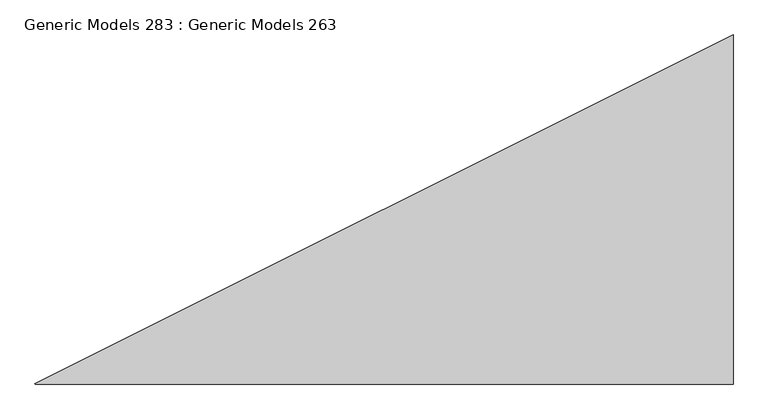
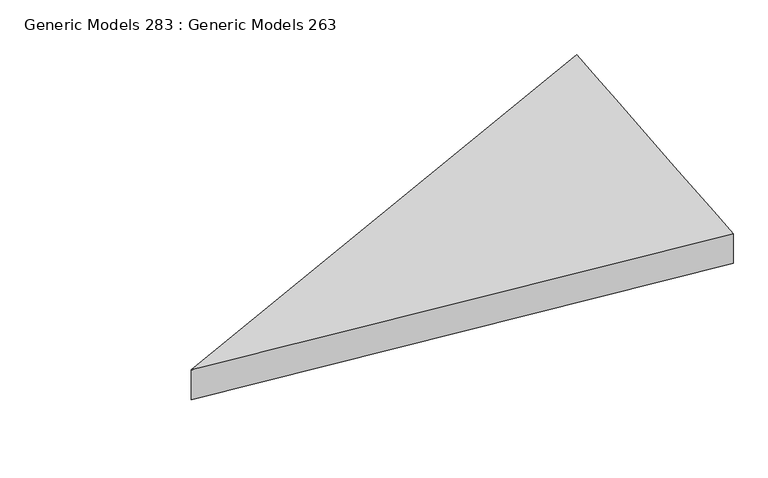
"""IFC4 building model written with IfcOpenShell, lengths in millimetres: proxy geometry, Generic Models 283 : Generic Models 263."""

from ifc_helpers import new_model, si_unit, frame, origin, place, context, project, spatial, source, transform, mapped, element, save
from ifc_brep_helpers import plane_surface, spline_surface, advanced_brep


def generic_models_283_generic_models_263_0de525de(model_context):
    return source(origin(), model_context, "Body", "AdvancedBrep", [
        advanced_brep(
        [(91554.5797726, 2106.5727422, 2.0699085), (91554.5797726, 582.5727422, -137.0198762), (91554.5797726, 582.5727422, -314.8198762), (91554.5797726, 2106.5727422, -314.8198762), (88506.5797726, 583.7192284, 120.3150753), (88506.5797726, 583.7192284, -58.1173502), (88506.5797726, 582.5727422, -58.1173502), (88506.5797726, 582.5727422, 120.3150753)],
        [
            (0, 1),
            (1, 2),
            (2, 3),
            (3, 0),
            (4, 5),
            (5, 6),
            (6, 7),
            (7, 4),
            (4, 0),
            (3, 5),
            (2, 6),
            (1, 7),
        ],
        [
            plane_surface(frame((91554.5797726, 1344.5727422, -191.14743), z_axis=(1.0, 0.0, 0.0), x_axis=(0.0, -0.9958610732446469, -0.09088851850492481))),
            plane_surface(frame((88506.5797726, 583.1459853, 31.0988625), z_axis=(-1.0, 0.0, 0.0), x_axis=(0.0, -0.9958610732446469, -0.09088851850492481))),
            plane_surface(frame((88506.5797726, 583.7192284, 31.0988625), z_axis=(-0.44694438819938226, 0.894561744016074, 0.0), x_axis=(0.0, 0.0, 1.0))),
            plane_surface(frame((88506.5797726, 583.1459853, -58.1173502), z_axis=(-0.08392288197547058, 0.0, -0.9964722524390387), x_axis=(0.0, 1.0, 0.0))),
            plane_surface(frame((88506.5797726, 582.5727422, 31.0988625), z_axis=(0.0, -1.0, 0.0), x_axis=(0.0, 0.0, -1.0))),
            spline_surface(1, 1, [[(88506.5797726, 583.7192284, 120.3150753), (91554.5797726, 2106.5727422, 2.0699085)], [(88506.5797726, 582.5727422, 120.3150753), (91554.5797726, 582.5727422, -137.0198762)]], [2, 2], [2, 2], [0.0, 1.0], [0.0, 1.0]),
        ],
        [
            (0, [[1, 2, 3, 4]]),
            (1, [[5, 6, 7, 8]]),
            (2, [[-5, 9, -4, 10]]),
            (3, [[-6, -10, -3, 11]]),
            (4, [[-7, -11, -2, 12]]),
            (5, [[-8, -12, -1, -9]]),
        ],
    ),
    ])


if __name__ == "__main__":
    model = new_model("IFC4")
    model_context = context("Model", 3, world=origin())
    ifc_project = project(units=[si_unit("LENGTHUNIT", "METRE", prefix="MILLI")], contexts=[model_context])
    site = spatial("IfcSite", under=ifc_project)
    building = spatial("IfcBuilding", under=site)
    placement = place(None, origin())
    generic_models_283_generic_models_263_shape = generic_models_283_generic_models_263_0de525de(model_context)
    element("IfcBuildingElementProxy", 1, Name="Generic Models 283 : Generic Models 263", ObjectType="Generic Models 283 : Generic Models 263", at=placement, inside=building, context=model_context, shape_type="MappedRepresentation", body=[
        mapped(generic_models_283_generic_models_263_shape, transform((0.0, 0.0, 0.0), x_axis=(1.0, 0.0, 0.0), y_axis=(0.0, 1.0, 0.0), z_axis=(0.0, 0.0, 1.0))),
    ])
    save(model, "model.ifc")

# Revit data of these elements
# Element 1 (IfcBuildingElementProxy, "Generic Models 283 : Generic Models 263")
#   Materials on its faces: "SLOPED - 7\" CONC."
# Materials
#   "SLOPED - 7\" CONC.": class "Concrete", colour RGB 191 191 191, transparency 0, Description = "Cast-in-place concrete", Cost = 0
